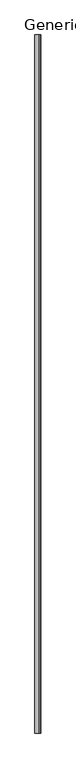
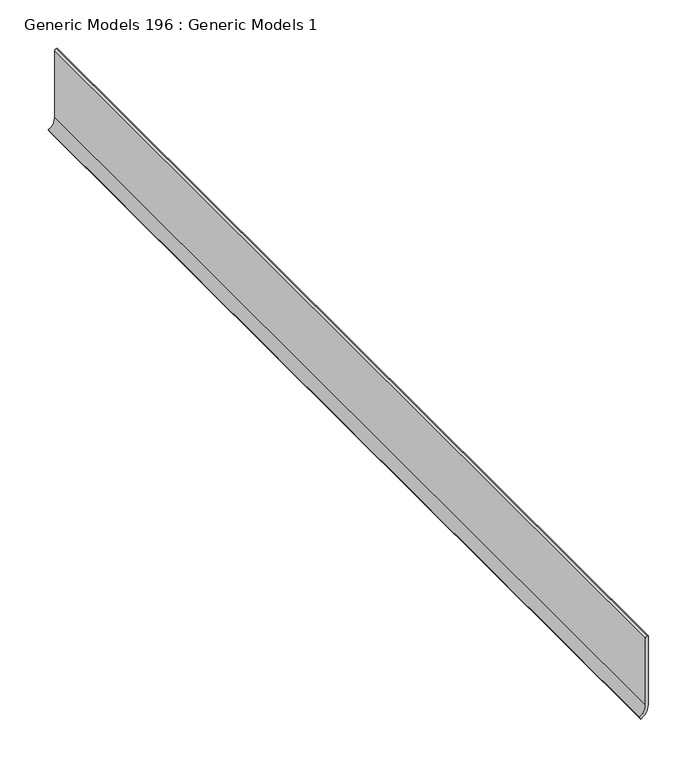
"""IFC4 building model written with IfcOpenShell, lengths in millimetres: proxy geometry, Generic Models 196 : Generic Models 1."""

from ifc_helpers import new_model, si_unit, point, frame, frame_2d, origin, place, context, project, spatial, polyline, circle_curve, trimmed, segment, composite_curve, outline, extrude, source, transform, mapped, element, save


def generic_models_196_generic_models_1_05ff5199(model_context):
    return source(origin(), model_context, "Body", "SweptSolid", [
        extrude(outline(composite_curve([segment(polyline([(-1822.8473206, 52542.4946108), (-1822.8473206, 52541.4064126)]), True, "CONTINUOUS"), segment(trimmed(circle_curve(frame_2d((-1824.9341224, 52541.4064126)), 2.0868018), [point((-1822.8473206, 52541.4064126))], [point((-1824.9341224, 52539.3196108))], False, "CARTESIAN"), True, "CONTINUOUS"), segment(polyline([(-1824.9341224, 52539.3196108), (-1908.9976899, 52539.3196108)]), True, "CONTINUOUS"), segment(trimmed(circle_curve(frame_2d((-1908.9976899, 52524.654914)), 14.6646968), [point((-1908.9976899, 52539.3196108))], [point((-1921.6976899, 52531.9872624))], True, "CARTESIAN"), True, "CONTINUOUS"), segment(polyline([(-1921.6976899, 52531.9872624), (-1924.4473206, 52533.5747624)]), True, "CONTINUOUS"), segment(trimmed(circle_curve(frame_2d((-1908.9976899, 52524.654914)), 17.8396968), [point((-1924.4473206, 52533.5747624))], [point((-1908.9976899, 52542.4946108))], False, "CARTESIAN"), True, "CONTINUOUS"), segment(polyline([(-1908.9976899, 52542.4946108), (-1822.8473206, 52542.4946108)]), True, "CONTINUOUS")], self_intersect=False)), frame((0.0, 0.0, 0.0), z_axis=(0.0, 1.0, 0.0), x_axis=(0.0, 0.0, 1.0)), (0.0, 0.0, 1.0), 1219.2),
    ])


if __name__ == "__main__":
    model = new_model("IFC4")
    model_context = context("Model", 3, world=origin())
    ifc_project = project(units=[si_unit("LENGTHUNIT", "METRE", prefix="MILLI")], contexts=[model_context])
    site = spatial("IfcSite", under=ifc_project)
    building = spatial("IfcBuilding", under=site)
    placement = place(None, origin())
    generic_models_196_generic_models_1_shape = generic_models_196_generic_models_1_05ff5199(model_context)
    element("IfcBuildingElementProxy", 1, Name="Generic Models 196 : Generic Models 1", ObjectType="Generic Models 196 : Generic Models 1", at=placement, inside=building, context=model_context, shape_type="MappedRepresentation", body=[
        mapped(generic_models_196_generic_models_1_shape, transform((0.0, 0.0, 0.0), x_axis=(1.0, 0.0, 0.0), y_axis=(0.0, 1.0, 0.0), z_axis=(0.0, 0.0, 1.0))),
    ])
    save(model, "model.ifc")

# Revit data of these elements
# Element 1 (IfcBuildingElementProxy, "Generic Models 196 : Generic Models 1")
#   Materials on its faces: "BASE T.B.D."
# Materials
#   "BASE T.B.D.": class "Generic", colour RGB 120 120 120, transparency 0, Cost = 0
